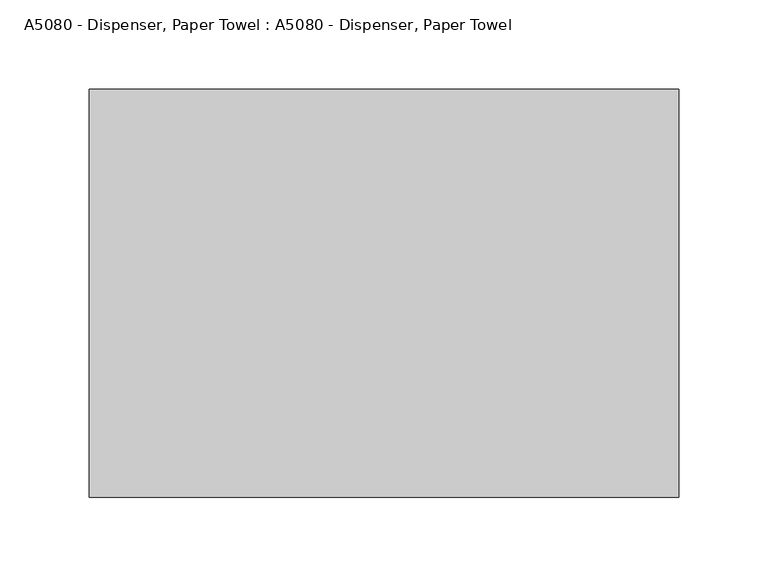
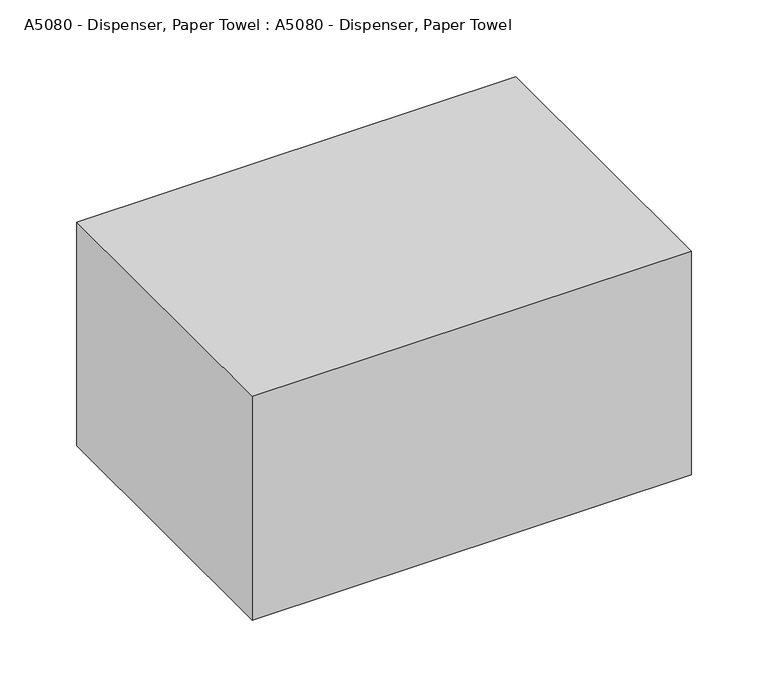
"""IFC4 building model written with IfcOpenShell, lengths in millimetres: proxy geometry, A5080 - Dispenser, Paper Towel : A5080 - Dispenser, Paper Towel."""

import ifcopenshell
import ifcopenshell.guid

model = None  # the IFC model being written
_history = None  # IfcOwnerHistory: only IFC2X3 demands one
_inside = {}  # id of a spatial element -> (the spatial element, [elements in it])
_under = {}  # id of a project, library or spatial element -> (it, [spatial elements below it])
_declared = {}  # id of a project -> (the project, [libraries it declares])
_typed = {}  # id of a type object -> (the type object, [elements of that type])
_made_of = {}  # id of a material, layer set ... -> (it, [elements and type objects made of it])


def new_model(schema):
    """Start an empty IFC model of exactly this schema.

    Asked for "IFC4X3", IfcOpenShell would pick the latest addendum, in which some entities
    have other attributes; the version numbers below select the first issue.
    IFC2X3 requires an IfcOwnerHistory on every rooted entity: one is made here for all.
    """
    global model, _history
    if schema == "IFC4X3":
        model = ifcopenshell.file(schema_version=(4, 3, 0, 0))
    else:
        model = ifcopenshell.file(schema=schema)
    _inside.clear()
    _under.clear()
    _declared.clear()
    _typed.clear()
    _made_of.clear()
    _history = None
    if model.schema == "IFC2X3":
        org = make("IfcOrganization", Name="unknown")
        user = make(
            "IfcPersonAndOrganization",
            ThePerson=make("IfcPerson", FamilyName="unknown"),
            TheOrganization=org,
        )
        app = make(
            "IfcApplication",
            ApplicationDeveloper=org,
            Version="unknown",
            ApplicationFullName="unknown",
            ApplicationIdentifier="unknown",
        )
        _history = make(
            "IfcOwnerHistory",
            OwningUser=user,
            OwningApplication=app,
            ChangeAction="ADDED",
            CreationDate=0,
        )
    return model


def make(cls, **values):
    """One entity of the class cls with the attributes given. An attribute that is None is left unset."""
    return model.create_entity(
        cls, **{name: value for name, value in values.items() if value is not None}
    )


def rooted(cls, **values):
    """An entity with a GlobalId (a new one), such as an element, a storey or a relation."""
    return make(cls, GlobalId=ifcopenshell.guid.new(), OwnerHistory=_history, **values)


def si_unit(unit_type, name, prefix=None):
    """IfcSIUnit, for example si_unit("LENGTHUNIT", "METRE", prefix="MILLI")."""
    return make("IfcSIUnit", UnitType=unit_type, Prefix=prefix, Name=name)


def assignment(units):
    """IfcUnitAssignment: the units of a project."""
    return None if units is None else make("IfcUnitAssignment", Units=units)


def point(xyz):
    """IfcCartesianPoint."""
    return None if xyz is None else make("IfcCartesianPoint", Coordinates=xyz)


def direction(xyz):
    """IfcDirection."""
    return None if xyz is None else make("IfcDirection", DirectionRatios=xyz)


def frame(location, z_axis=None, x_axis=None):
    """IfcAxis2Placement3D, a coordinate frame: its origin and axes. An axis left out is left unset."""
    return make(
        "IfcAxis2Placement3D",
        Location=point(location),
        Axis=direction(z_axis),
        RefDirection=direction(x_axis),
    )


def origin():
    """The frame at (0, 0, 0) with its axes left unset."""
    return frame((0.0, 0.0, 0.0))


def origin_with_axes():
    """The frame at (0, 0, 0) with the z axis (0, 0, 1) and the x axis (1, 0, 0) written out."""
    return frame((0.0, 0.0, 0.0), z_axis=(0.0, 0.0, 1.0), x_axis=(1.0, 0.0, 0.0))


def place(relative_to, where):
    """IfcLocalPlacement: puts the frame where relative to a parent placement (None: the world)."""
    return make(
        "IfcLocalPlacement", PlacementRelTo=relative_to, RelativePlacement=where
    )


def context(
    kind, dimensions, precision=None, world=None, true_north=None, identifier=None
):
    """IfcGeometricRepresentationContext, for example the 3D "Model" context."""
    return make(
        "IfcGeometricRepresentationContext",
        ContextIdentifier=identifier,
        ContextType=kind,
        CoordinateSpaceDimension=dimensions,
        Precision=precision,
        WorldCoordinateSystem=world,
        TrueNorth=true_north,
    )


def project(units=None, contexts=None):
    """IfcProject with its units and contexts."""
    return rooted(
        "IfcProject",
        Name="project",
        RepresentationContexts=contexts,
        UnitsInContext=assignment(units),
    )


def spatial(cls, under=None, at=None, **own):
    """A site, building, storey or space (cls), placed at a placement, below another one or the project."""
    s = rooted(cls, ObjectPlacement=at, **own)
    if under is not None:
        _under.setdefault(under.id(), (under, []))[1].append(s)
    return s


def polyline(points):
    """IfcPolyline through the points."""
    return make("IfcPolyline", Points=[point(p) for p in points])


def outline(outer, holes=None, kind="AREA"):
    """IfcArbitraryClosedProfileDef: a profile drawn as a closed curve; with holes, ...WithVoids."""
    if holes is None:
        return make("IfcArbitraryClosedProfileDef", ProfileType=kind, OuterCurve=outer)
    return make(
        "IfcArbitraryProfileDefWithVoids",
        ProfileType=kind,
        OuterCurve=outer,
        InnerCurves=holes,
    )


def extrude(swept, where, along, depth):
    """IfcExtrudedAreaSolid: the profile swept, set in the frame where, extruded along a direction by depth."""
    return make(
        "IfcExtrudedAreaSolid",
        SweptArea=swept,
        Position=where,
        ExtrudedDirection=direction(along),
        Depth=depth,
    )


def shape(context_of_items, identifier, shape_type, items):
    """IfcShapeRepresentation: the items that make up one representation, for example the "Body"."""
    return make(
        "IfcShapeRepresentation",
        ContextOfItems=context_of_items,
        RepresentationIdentifier=identifier,
        RepresentationType=shape_type,
        Items=items,
    )


def source(mapping_origin, context_of_items, identifier, shape_type, items):
    """IfcRepresentationMap: a shape defined once, which mapped items show again and again."""
    return make(
        "IfcRepresentationMap",
        MappingOrigin=mapping_origin,
        MappedRepresentation=shape(context_of_items, identifier, shape_type, items),
    )


def transform(
    local_origin,
    x_axis=None,
    y_axis=None,
    z_axis=None,
    scale=None,
    scale2=None,
    scale3=None,
    uniform=True,
):
    """IfcCartesianTransformationOperator3D, or its non-uniform kind. x_axis, y_axis, z_axis: its Axis1, 2, 3."""
    if uniform:
        return make(
            "IfcCartesianTransformationOperator3D",
            Axis1=direction(x_axis),
            Axis2=direction(y_axis),
            LocalOrigin=point(local_origin),
            Scale=scale,
            Axis3=direction(z_axis),
        )
    return make(
        "IfcCartesianTransformationOperator3DnonUniform",
        Axis1=direction(x_axis),
        Axis2=direction(y_axis),
        LocalOrigin=point(local_origin),
        Scale=scale,
        Axis3=direction(z_axis),
        Scale2=scale2,
        Scale3=scale3,
    )


def mapped(mapping_source, mapping_target):
    """IfcMappedItem: shows the shape of a source again, moved by a transform."""
    return make(
        "IfcMappedItem", MappingSource=mapping_source, MappingTarget=mapping_target
    )


def made_of(thing, what):
    """Note that an element or type object is made of a material, layer set ...; save() writes the relation."""
    if what is not None:
        _made_of.setdefault(what.id(), (what, []))[1].append(thing)
    return thing


def element(
    cls,
    number,
    at=None,
    inside=None,
    cuts=None,
    type_object=None,
    material=None,
    context=None,
    identifier="Body",
    shape_type=None,
    held_by="IfcProductDefinitionShape",
    body=None,
    shapes=None,
    **own,
):
    """One element of the class cls, such as IfcWall. Its Tag is "e" and its number.

    at: its placement. inside: the storey or other place that contains it. cuts: it is an
    opening in that element (IfcRelVoidsElement). A single representation is given by context,
    identifier, shape_type and body (its items); several are given by shapes. held_by: the class
    of the entity that holds the representations. save() writes the other relations.
    """
    e = rooted(cls, Tag="e%d" % number, ObjectPlacement=at, **own)
    if body is not None:
        shapes = [shape(context, identifier, shape_type, body)]
    if shapes is not None:
        e.Representation = make(held_by, Representations=shapes)
    if inside is not None:
        _inside.setdefault(inside.id(), (inside, []))[1].append(e)
    if cuts is not None:
        rooted(
            "IfcRelVoidsElement", RelatingBuildingElement=cuts, RelatedOpeningElement=e
        )
    if type_object is not None:
        _typed.setdefault(type_object.id(), (type_object, []))[1].append(e)
    return made_of(e, material)


def aggregate(whole, parts):
    """IfcRelAggregates: a whole, such as a stair, and the parts it consists of."""
    return rooted("IfcRelAggregates", RelatingObject=whole, RelatedObjects=parts)


def save(model, path):
    """Write the relations noted so far, then the file.

    IfcRelAggregates (storeys below a building ...), IfcRelContainedInSpatialStructure (elements
    in a storey), IfcRelDefinesByType, IfcRelAssociatesMaterial and IfcRelDeclares: one each for
    every whole, place, type object, material and project.
    """
    for whole, parts in _under.values():
        aggregate(whole, parts)
    for where, things in _inside.values():
        rooted(
            "IfcRelContainedInSpatialStructure",
            RelatedElements=things,
            RelatingStructure=where,
        )
    for kind, things in _typed.values():
        rooted("IfcRelDefinesByType", RelatedObjects=things, RelatingType=kind)
    for what, things in _made_of.values():
        rooted("IfcRelAssociatesMaterial", RelatedObjects=things, RelatingMaterial=what)
    for by, libraries in _declared.values():
        rooted("IfcRelDeclares", RelatingContext=by, RelatedDefinitions=libraries)
    model.write(path)


def a5080_dispenser_paper_towel_a5080_dispenser_paper_towel_61bbfe70(model_context):
    return source(origin(), model_context, "Body", "SweptSolid", [
        extrude(outline(polyline([(165.1, 228.6), (165.1, 0.0), (-165.1, 0.0), (-165.1, 228.6), (165.1, 228.6)])), origin_with_axes(), (0.0, 0.0, 1.0), 177.8),
        extrude(outline(polyline([(-165.1, 228.6), (165.1, 228.6), (165.1, 0.0), (-165.1, 0.0), (-165.1, 228.6)])), origin_with_axes(), (0.0, 0.0, 1.0), 177.8),
    ])


if __name__ == "__main__":
    model = new_model("IFC4")
    model_context = context("Model", 3, world=origin())
    ifc_project = project(units=[si_unit("LENGTHUNIT", "METRE", prefix="MILLI")], contexts=[model_context])
    site = spatial("IfcSite", under=ifc_project)
    building = spatial("IfcBuilding", under=site)
    placement = place(None, origin())
    a5080_dispenser_paper_towel_a5080_dispenser_paper_towel_shape = a5080_dispenser_paper_towel_a5080_dispenser_paper_towel_61bbfe70(model_context)
    element("IfcBuildingElementProxy", 1, Name="A5080 - Dispenser, Paper Towel : A5080 - Dispenser, Paper Towel", ObjectType="A5080 - Dispenser, Paper Towel : A5080 - Dispenser, Paper Towel", at=placement, inside=building, context=model_context, shape_type="MappedRepresentation", body=[
        mapped(a5080_dispenser_paper_towel_a5080_dispenser_paper_towel_shape, transform((0.0, 0.0, 0.0), x_axis=(1.0, 0.0, 0.0), y_axis=(0.0, 1.0, 0.0), z_axis=(0.0, 0.0, 1.0))),
    ])
    save(model, "model.ifc")

# Revit data of these elements
# Type "A5080 - Dispenser, Paper Towel : A5080 - Dispenser, Paper Towel"
#   Watts2 = "0"
#   Watts1 = "0"
#   Unit_Issue = "EA"
#   UTIL_6_Misc = "-"
#   UTIL_5_NonMedGas = "-"
#   UTIL_4_MiscGas = "-"
#   UTIL_3_MedGas = "-"
#   UTIL_2_Elec = "-"
#   UTIL_1_WaterDrain = "-"
#   Nomenclature = "Dispenser, Paper Towel, SS, Surface Mounted"
#   NSN = "4510"
#   Location [instance default] = ""
#   JSN = "A5080"
#   Fund_Source_VA = "-"
#   Fund_Source_Navy = "-"
#   Fund_Source_Army = "-"
#   Fund_Source_AF = "-"
#   ELEC_Volts2 = "0"
#   ELEC_Volts1 = "0"
#   ELEC_Phase2 = "0"
#   ELEC_Phase1 = "0"
#   ELEC_HertzSwitch = "0"
#   ELEC_HertzDependent = "0"
#   ELEC_Hertz = "0"
#   ELEC_Amps2 = "0"
#   ELEC_Amps1 = "0"
#   DetailDescription = "A surface mounted, satin finish stainless steel, single-fold, paper towel dispenser. Dispenser features: tumbler lock; front hinged at bottom; and refill indicator slot. Minimum capacity 400 single-fold paper towels. For general purpose use throughout the facility."
#   CAT_VA = "A"
#   CAT_Navy = "A"
#   CAT_IHS = "-"
#   CAT_Army = "A"
#   CAT_AF = "A"
#   BTUperhour = "0"
#   Weight_IP = 4
#   Default Elevation = 4' - 0"
#   DIM_Width_IP = 1' - 1"
#   DIM_Height_IP = 0' - 9"
#   DIM_Depth_IP = 0' - 7"
#   Assembly Code = ""
# Element 1 (IfcBuildingElementProxy, "A5080 - Dispenser, Paper Towel : A5080 - Dispenser, Paper Towel")
#   Location = "TRET3"
#   Materials on its faces: "EquipSpace", "Wall Material (1)"
# Materials
#   "EquipSpace": class "Unassigned", colour RGB 221 217 195, transparency 0.5
#   "Wall Material (1)": class "Miscellaneous", colour RGB 234 233 232, transparency 0
